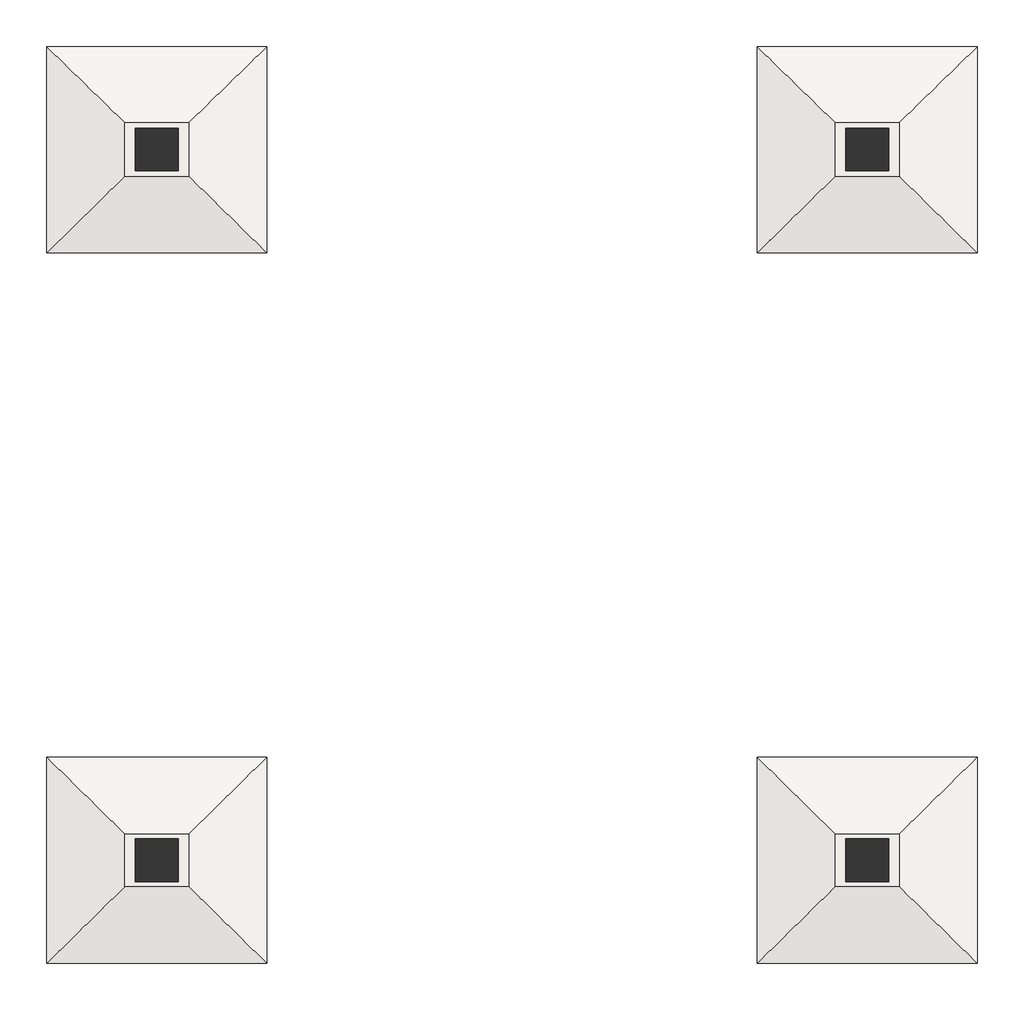
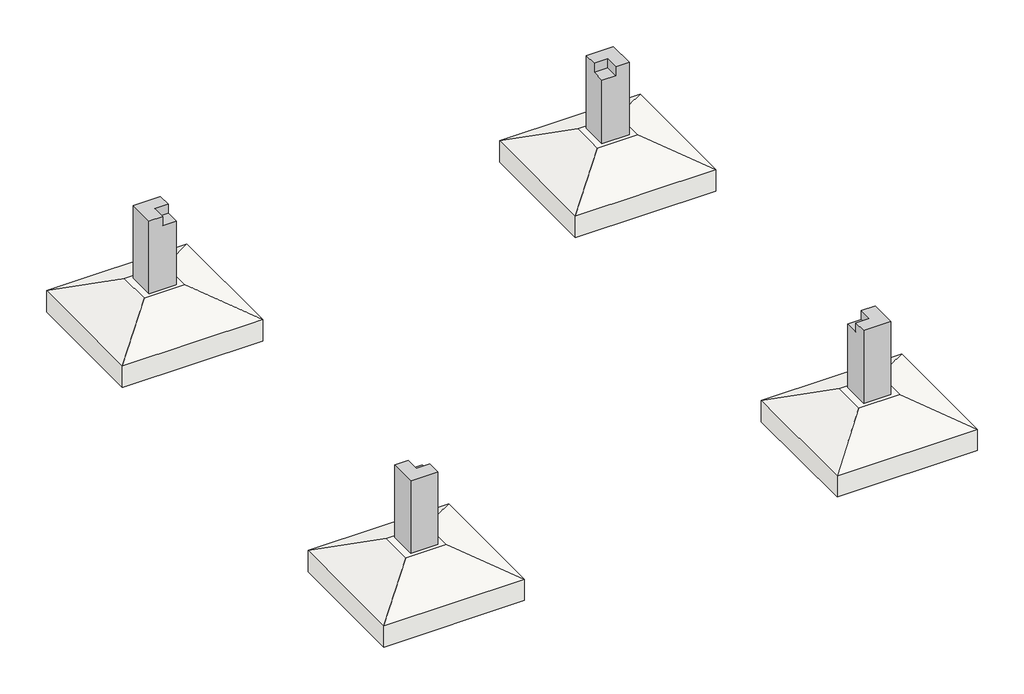
# One storey: 4 columns, 4 slabs.
"""IFC4 building model written with IfcOpenShell, lengths in millimetres."""

from ifc_helpers import new_model, si_unit, origin, place, context, project, spatial, faceted_brep, element, save

model = new_model("IFC4")

# Units and contexts
model_context = context("Model", 3, world=origin())
ifc_project = project(units=[si_unit("LENGTHUNIT", "METRE", prefix="MILLI")], contexts=[model_context])

# Site, building, storey
site = spatial("IfcSite", under=ifc_project)
building = spatial("IfcBuilding", under=site)
storey = spatial("IfcBuildingStorey", under=building, Name="Fundação", Elevation=-1700.0)

# Columns
placement = place(None, origin())
element("IfcColumn", 1, ObjectType="Concreto-Quadrado-Coluna : 600 x 600mm", at=placement, inside=storey, context=model_context, shape_type="Brep", body=[
    faceted_brep([(-2623.6821965, 6511.329614, -1700.0), (-2623.6821965, 5911.329614, -1700.0), (-3223.6821965, 5911.329614, -1700.0), (-3223.6821965, 6511.329614, -1700.0), (-2623.6821965, 6511.329614, 0.0), (-2623.6821965, 6211.329614, 0.0), (-2623.6821965, 6211.329614, -210.0), (-2623.6821965, 5911.329614, -210.0), (-2923.6821965, 5911.329614, -210.0), (-2923.6821965, 5911.329614, 0.0), (-3223.6821965, 5911.329614, 0.0), (-3223.6821965, 6511.329614, 0.0), (-2923.6821965, 6211.329614, 0.0), (-2923.6821965, 6211.329614, -210.0)], [[[0, 1, 2, 3]], [[1, 0, 4, 5, 6, 7]], [[2, 1, 7, 8, 9, 10]], [[3, 2, 10, 11]], [[0, 3, 11, 4]], [[11, 10, 9, 12, 5, 4]], [[6, 13, 8, 7]], [[13, 12, 9, 8]], [[12, 13, 6, 5]]]),
])
element("IfcColumn", 2, ObjectType="Concreto-Quadrado-Coluna : 600 x 600mm", at=placement, inside=storey, context=model_context, shape_type="Brep", body=[
    faceted_brep([(7376.3178035, 6511.329614, -1700.0), (7376.3178035, 5911.329614, -1700.0), (6776.3178035, 5911.329614, -1700.0), (6776.3178035, 6511.329614, -1700.0), (7376.3178035, 6511.329614, 0.0), (7376.3178035, 5911.329614, 0.0), (7076.3178035, 5911.329614, 0.0), (7076.3178035, 5911.329614, -210.0), (6776.3178035, 5911.329614, -210.0), (6776.3178035, 6211.329614, -210.0), (6776.3178035, 6211.329614, 0.0), (6776.3178035, 6511.329614, 0.0), (7076.3178035, 6211.329614, 0.0), (7076.3178035, 6211.329614, -210.0)], [[[0, 1, 2, 3]], [[1, 0, 4, 5]], [[2, 1, 5, 6, 7, 8]], [[3, 2, 8, 9, 10, 11]], [[0, 3, 11, 4]], [[5, 4, 11, 10, 12, 6]], [[13, 9, 8, 7]], [[12, 13, 7, 6]], [[13, 12, 10, 9]]]),
])
element("IfcColumn", 3, ObjectType="Concreto-Quadrado-Coluna : 600 x 600mm", at=placement, inside=storey, context=model_context, shape_type="Brep", body=[
    faceted_brep([(7376.3178035, -3488.670386, -1700.0), (7376.3178035, -4088.670386, -1700.0), (6776.3178035, -4088.670386, -1700.0), (6776.3178035, -3488.670386, -1700.0), (7376.3178035, -3488.670386, 0.0), (7376.3178035, -4088.670386, 0.0), (6776.3178035, -4088.670386, 0.0), (6776.3178035, -3788.670386, 0.0), (6776.3178035, -3788.670386, -210.0), (6776.3178035, -3488.670386, -210.0), (7076.3178035, -3488.670386, -210.0), (7076.3178035, -3488.670386, 0.0), (7076.3178035, -3788.670386, 0.0), (7076.3178035, -3788.670386, -210.0)], [[[0, 1, 2, 3]], [[1, 0, 4, 5]], [[2, 1, 5, 6]], [[3, 2, 6, 7, 8, 9]], [[0, 3, 9, 10, 11, 4]], [[5, 4, 11, 12, 7, 6]], [[8, 13, 10, 9]], [[13, 12, 11, 10]], [[12, 13, 8, 7]]]),
])
element("IfcColumn", 4, ObjectType="Concreto-Quadrado-Coluna : 600 x 600mm", at=placement, inside=storey, context=model_context, shape_type="Brep", body=[
    faceted_brep([(-2623.6821965, -3488.670386, -1700.0), (-2623.6821965, -4088.670386, -1700.0), (-3223.6821965, -4088.670386, -1700.0), (-3223.6821965, -3488.670386, -1700.0), (-2623.6821965, -3488.670386, -210.0), (-2623.6821965, -3788.670386, -210.0), (-2623.6821965, -3788.670386, 0.0), (-2623.6821965, -4088.670386, 0.0), (-3223.6821965, -4088.670386, 0.0), (-3223.6821965, -3488.670386, 0.0), (-2923.6821965, -3488.670386, 0.0), (-2923.6821965, -3488.670386, -210.0), (-2923.6821965, -3788.670386, 0.0), (-2923.6821965, -3788.670386, -210.0)], [[[0, 1, 2, 3]], [[1, 0, 4, 5, 6, 7]], [[2, 1, 7, 8]], [[3, 2, 8, 9]], [[0, 3, 9, 10, 11, 4]], [[8, 7, 6, 12, 10, 9]], [[11, 13, 5, 4]], [[13, 12, 6, 5]], [[12, 13, 11, 10]]]),
])

# Slabs
element("IfcSlab", 5, ObjectType="Sapata distribuída - Cônica : 3100x2900x1050", at=placement, inside=storey, context=model_context, shape_type="Brep", body=[
    faceted_brep([(-1373.6821965, 7661.329614, -2750.0), (-1373.6821965, 4761.329614, -2750.0), (-4473.6821965, 4761.329614, -2750.0), (-4473.6821965, 7661.329614, -2750.0), (-4473.6821965, 7661.329614, -2250.0), (-1373.6821965, 7661.329614, -2250.0), (-4473.6821965, 4761.329614, -2250.0), (-1373.6821965, 4761.329614, -2250.0), (-2473.6821965, 6586.329614, -1700.0), (-3373.6821965, 6586.329614, -1700.0), (-3373.6821965, 5836.329614, -1700.0), (-2473.6821965, 5836.329614, -1700.0)], [[[0, 1, 2, 3]], [[0, 3, 4, 5]], [[3, 2, 6, 4]], [[2, 1, 7, 6]], [[1, 0, 5, 7]], [[8, 9, 10, 11]], [[9, 8, 5, 4]], [[10, 9, 4, 6]], [[11, 10, 6, 7]], [[8, 11, 7, 5]]]),
])
element("IfcSlab", 6, ObjectType="Sapata distribuída - Cônica : 3100x2900x1050", at=placement, inside=storey, context=model_context, shape_type="Brep", body=[
    faceted_brep([(8626.3178035, 7661.329614, -2750.0), (8626.3178035, 4761.329614, -2750.0), (5526.3178035, 4761.329614, -2750.0), (5526.3178035, 7661.329614, -2750.0), (5526.3178035, 7661.329614, -2250.0), (8626.3178035, 7661.329614, -2250.0), (5526.3178035, 4761.329614, -2250.0), (8626.3178035, 4761.329614, -2250.0), (7526.3178035, 6586.329614, -1700.0), (6626.3178035, 6586.329614, -1700.0), (6626.3178035, 5836.329614, -1700.0), (7526.3178035, 5836.329614, -1700.0)], [[[0, 1, 2, 3]], [[0, 3, 4, 5]], [[3, 2, 6, 4]], [[2, 1, 7, 6]], [[1, 0, 5, 7]], [[8, 9, 10, 11]], [[9, 8, 5, 4]], [[10, 9, 4, 6]], [[11, 10, 6, 7]], [[8, 11, 7, 5]]]),
])
element("IfcSlab", 7, ObjectType="Sapata distribuída - Cônica : 3100x2900x1050", at=placement, inside=storey, context=model_context, shape_type="Brep", body=[
    faceted_brep([(8626.3178035, -2338.670386, -2750.0), (8626.3178035, -5238.670386, -2750.0), (5526.3178035, -5238.670386, -2750.0), (5526.3178035, -2338.670386, -2750.0), (5526.3178035, -2338.670386, -2250.0), (8626.3178035, -2338.670386, -2250.0), (5526.3178035, -5238.670386, -2250.0), (8626.3178035, -5238.670386, -2250.0), (7526.3178035, -3413.670386, -1700.0), (6626.3178035, -3413.670386, -1700.0), (6626.3178035, -4163.670386, -1700.0), (7526.3178035, -4163.670386, -1700.0)], [[[0, 1, 2, 3]], [[0, 3, 4, 5]], [[3, 2, 6, 4]], [[2, 1, 7, 6]], [[1, 0, 5, 7]], [[8, 9, 10, 11]], [[9, 8, 5, 4]], [[10, 9, 4, 6]], [[11, 10, 6, 7]], [[8, 11, 7, 5]]]),
])
element("IfcSlab", 8, ObjectType="Sapata distribuída - Cônica : 3100x2900x1050", at=placement, inside=storey, context=model_context, shape_type="Brep", body=[
    faceted_brep([(-1373.6821965, -2338.670386, -2750.0), (-1373.6821965, -5238.670386, -2750.0), (-4473.6821965, -5238.670386, -2750.0), (-4473.6821965, -2338.670386, -2750.0), (-4473.6821965, -2338.670386, -2250.0), (-1373.6821965, -2338.670386, -2250.0), (-4473.6821965, -5238.670386, -2250.0), (-1373.6821965, -5238.670386, -2250.0), (-2473.6821965, -3413.670386, -1700.0), (-3373.6821965, -3413.670386, -1700.0), (-3373.6821965, -4163.670386, -1700.0), (-2473.6821965, -4163.670386, -1700.0)], [[[0, 1, 2, 3]], [[0, 3, 4, 5]], [[3, 2, 6, 4]], [[2, 1, 7, 6]], [[1, 0, 5, 7]], [[8, 9, 10, 11]], [[9, 8, 5, 4]], [[10, 9, 4, 6]], [[11, 10, 6, 7]], [[8, 11, 7, 5]]]),
])

save(model, "model.ifc")

# Revit data of these elements
# Project information
#   Data de emissão do projeto = "Data de emissão"
#   Status do projeto = "Status do projeto"
#   Nome do cliente = "Proprietário"
#   Endereço do projeto = "Insira aqui o endereço"
#   Nome do projeto = "Nome do projeto"
#   Número do projeto = "0001"
# Grids (mm)
#   "1": line (-2923.682, 11218.77) -> (-2923.682, -10697.854)
#   "2": line (7076.318, 11218.77) -> (7076.318, -10697.854)
#   "3": line (-9963.128, 6211.33) -> (14493.503, 6211.33)
#   "4": line (-9963.128, -3788.67) -> (14493.503, -3788.67)
# Type "Concreto-Quadrado-Coluna : 600 x 600mm"
#   b = 0.60 m
#   Structural Material [instance default] = Concreto, Moldado in loco, cinza
# Type "Sapata distribuída - Cônica : 3100x2900x1050"
#   h1 = 0.50 m
#   Width = 3.10 m
#   Length = 2.90 m
#   L1 = 0.75 m
#   Foundation Thickness = 1.05 m
#   B1 = 0.90 m
#   Structural Material [instance default] = Concreto - Concreto moldado in loco
#   Assembly Code = ""
# Elements 1, 2, 3, 4 (IfcColumn, "Concreto-Quadrado-Coluna : 600 x 600mm")
#   Structural Material = Concreto, Moldado in loco, cinza
#   Phase Created = Construção nova
#   Materials on its faces: "Concreto, Moldado in loco, cinza"
# Elements 5, 6, 7, 8 (IfcSlab, "Sapata distribuída - Cônica : 3100x2900x1050")
#   Structural Material = Concreto - Concreto moldado in loco
#   Phase Created = Construção nova
#   Materials on its faces: "Concreto - Concreto moldado in loco"
# Materials
#   "Concreto, Moldado in loco, cinza": class "Concreto", colour RGB 192 192 192, transparency 0, Description = "Concreto moldado in loco", Cost = 0
#   "Concreto - Concreto moldado in loco": class "Concreto", colour RGB 192 192 192, transparency 0
